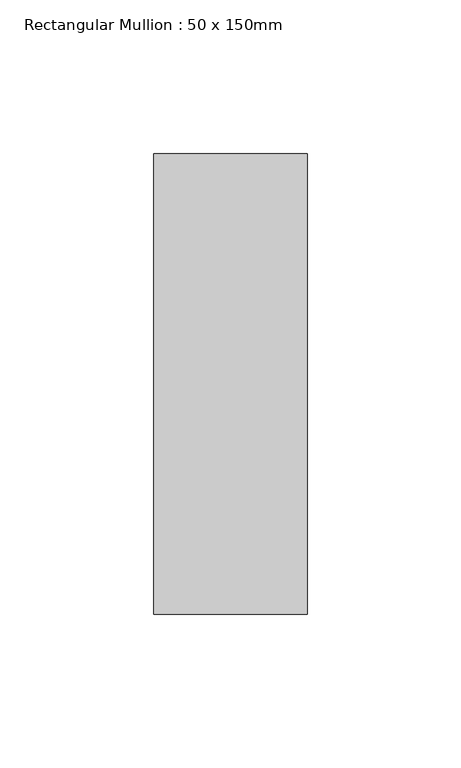
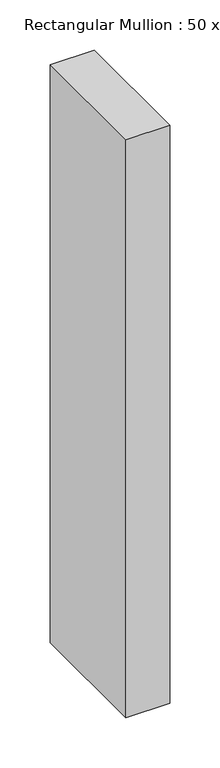
"""IFC4 building model written with IfcOpenShell, lengths in millimetres: member geometry, Rectangular Mullion : 50 x 150mm."""

import ifcopenshell
import ifcopenshell.guid

model = None  # the IFC model being written
_history = None  # IfcOwnerHistory: only IFC2X3 demands one
_inside = {}  # id of a spatial element -> (the spatial element, [elements in it])
_under = {}  # id of a project, library or spatial element -> (it, [spatial elements below it])
_declared = {}  # id of a project -> (the project, [libraries it declares])
_typed = {}  # id of a type object -> (the type object, [elements of that type])
_made_of = {}  # id of a material, layer set ... -> (it, [elements and type objects made of it])


def new_model(schema):
    """Start an empty IFC model of exactly this schema.

    Asked for "IFC4X3", IfcOpenShell would pick the latest addendum, in which some entities
    have other attributes; the version numbers below select the first issue.
    IFC2X3 requires an IfcOwnerHistory on every rooted entity: one is made here for all.
    """
    global model, _history
    if schema == "IFC4X3":
        model = ifcopenshell.file(schema_version=(4, 3, 0, 0))
    else:
        model = ifcopenshell.file(schema=schema)
    _inside.clear()
    _under.clear()
    _declared.clear()
    _typed.clear()
    _made_of.clear()
    _history = None
    if model.schema == "IFC2X3":
        org = make("IfcOrganization", Name="unknown")
        user = make(
            "IfcPersonAndOrganization",
            ThePerson=make("IfcPerson", FamilyName="unknown"),
            TheOrganization=org,
        )
        app = make(
            "IfcApplication",
            ApplicationDeveloper=org,
            Version="unknown",
            ApplicationFullName="unknown",
            ApplicationIdentifier="unknown",
        )
        _history = make(
            "IfcOwnerHistory",
            OwningUser=user,
            OwningApplication=app,
            ChangeAction="ADDED",
            CreationDate=0,
        )
    return model


def make(cls, **values):
    """One entity of the class cls with the attributes given. An attribute that is None is left unset."""
    return model.create_entity(
        cls, **{name: value for name, value in values.items() if value is not None}
    )


def rooted(cls, **values):
    """An entity with a GlobalId (a new one), such as an element, a storey or a relation."""
    return make(cls, GlobalId=ifcopenshell.guid.new(), OwnerHistory=_history, **values)


def si_unit(unit_type, name, prefix=None):
    """IfcSIUnit, for example si_unit("LENGTHUNIT", "METRE", prefix="MILLI")."""
    return make("IfcSIUnit", UnitType=unit_type, Prefix=prefix, Name=name)


def assignment(units):
    """IfcUnitAssignment: the units of a project."""
    return None if units is None else make("IfcUnitAssignment", Units=units)


def point(xyz):
    """IfcCartesianPoint."""
    return None if xyz is None else make("IfcCartesianPoint", Coordinates=xyz)


def direction(xyz):
    """IfcDirection."""
    return None if xyz is None else make("IfcDirection", DirectionRatios=xyz)


def frame(location, z_axis=None, x_axis=None):
    """IfcAxis2Placement3D, a coordinate frame: its origin and axes. An axis left out is left unset."""
    return make(
        "IfcAxis2Placement3D",
        Location=point(location),
        Axis=direction(z_axis),
        RefDirection=direction(x_axis),
    )


def origin():
    """The frame at (0, 0, 0) with its axes left unset."""
    return frame((0.0, 0.0, 0.0))


def place(relative_to, where):
    """IfcLocalPlacement: puts the frame where relative to a parent placement (None: the world)."""
    return make(
        "IfcLocalPlacement", PlacementRelTo=relative_to, RelativePlacement=where
    )


def context(
    kind, dimensions, precision=None, world=None, true_north=None, identifier=None
):
    """IfcGeometricRepresentationContext, for example the 3D "Model" context."""
    return make(
        "IfcGeometricRepresentationContext",
        ContextIdentifier=identifier,
        ContextType=kind,
        CoordinateSpaceDimension=dimensions,
        Precision=precision,
        WorldCoordinateSystem=world,
        TrueNorth=true_north,
    )


def project(units=None, contexts=None):
    """IfcProject with its units and contexts."""
    return rooted(
        "IfcProject",
        Name="project",
        RepresentationContexts=contexts,
        UnitsInContext=assignment(units),
    )


def spatial(cls, under=None, at=None, **own):
    """A site, building, storey or space (cls), placed at a placement, below another one or the project."""
    s = rooted(cls, ObjectPlacement=at, **own)
    if under is not None:
        _under.setdefault(under.id(), (under, []))[1].append(s)
    return s


def polyline(points):
    """IfcPolyline through the points."""
    return make("IfcPolyline", Points=[point(p) for p in points])


def outline(outer, holes=None, kind="AREA"):
    """IfcArbitraryClosedProfileDef: a profile drawn as a closed curve; with holes, ...WithVoids."""
    if holes is None:
        return make("IfcArbitraryClosedProfileDef", ProfileType=kind, OuterCurve=outer)
    return make(
        "IfcArbitraryProfileDefWithVoids",
        ProfileType=kind,
        OuterCurve=outer,
        InnerCurves=holes,
    )


def extrude(swept, where, along, depth):
    """IfcExtrudedAreaSolid: the profile swept, set in the frame where, extruded along a direction by depth."""
    return make(
        "IfcExtrudedAreaSolid",
        SweptArea=swept,
        Position=where,
        ExtrudedDirection=direction(along),
        Depth=depth,
    )


def shape(context_of_items, identifier, shape_type, items):
    """IfcShapeRepresentation: the items that make up one representation, for example the "Body"."""
    return make(
        "IfcShapeRepresentation",
        ContextOfItems=context_of_items,
        RepresentationIdentifier=identifier,
        RepresentationType=shape_type,
        Items=items,
    )


def source(mapping_origin, context_of_items, identifier, shape_type, items):
    """IfcRepresentationMap: a shape defined once, which mapped items show again and again."""
    return make(
        "IfcRepresentationMap",
        MappingOrigin=mapping_origin,
        MappedRepresentation=shape(context_of_items, identifier, shape_type, items),
    )


def transform(
    local_origin,
    x_axis=None,
    y_axis=None,
    z_axis=None,
    scale=None,
    scale2=None,
    scale3=None,
    uniform=True,
):
    """IfcCartesianTransformationOperator3D, or its non-uniform kind. x_axis, y_axis, z_axis: its Axis1, 2, 3."""
    if uniform:
        return make(
            "IfcCartesianTransformationOperator3D",
            Axis1=direction(x_axis),
            Axis2=direction(y_axis),
            LocalOrigin=point(local_origin),
            Scale=scale,
            Axis3=direction(z_axis),
        )
    return make(
        "IfcCartesianTransformationOperator3DnonUniform",
        Axis1=direction(x_axis),
        Axis2=direction(y_axis),
        LocalOrigin=point(local_origin),
        Scale=scale,
        Axis3=direction(z_axis),
        Scale2=scale2,
        Scale3=scale3,
    )


def mapped(mapping_source, mapping_target):
    """IfcMappedItem: shows the shape of a source again, moved by a transform."""
    return make(
        "IfcMappedItem", MappingSource=mapping_source, MappingTarget=mapping_target
    )


def made_of(thing, what):
    """Note that an element or type object is made of a material, layer set ...; save() writes the relation."""
    if what is not None:
        _made_of.setdefault(what.id(), (what, []))[1].append(thing)
    return thing


def element(
    cls,
    number,
    at=None,
    inside=None,
    cuts=None,
    type_object=None,
    material=None,
    context=None,
    identifier="Body",
    shape_type=None,
    held_by="IfcProductDefinitionShape",
    body=None,
    shapes=None,
    **own,
):
    """One element of the class cls, such as IfcWall. Its Tag is "e" and its number.

    at: its placement. inside: the storey or other place that contains it. cuts: it is an
    opening in that element (IfcRelVoidsElement). A single representation is given by context,
    identifier, shape_type and body (its items); several are given by shapes. held_by: the class
    of the entity that holds the representations. save() writes the other relations.
    """
    e = rooted(cls, Tag="e%d" % number, ObjectPlacement=at, **own)
    if body is not None:
        shapes = [shape(context, identifier, shape_type, body)]
    if shapes is not None:
        e.Representation = make(held_by, Representations=shapes)
    if inside is not None:
        _inside.setdefault(inside.id(), (inside, []))[1].append(e)
    if cuts is not None:
        rooted(
            "IfcRelVoidsElement", RelatingBuildingElement=cuts, RelatedOpeningElement=e
        )
    if type_object is not None:
        _typed.setdefault(type_object.id(), (type_object, []))[1].append(e)
    return made_of(e, material)


def aggregate(whole, parts):
    """IfcRelAggregates: a whole, such as a stair, and the parts it consists of."""
    return rooted("IfcRelAggregates", RelatingObject=whole, RelatedObjects=parts)


def save(model, path):
    """Write the relations noted so far, then the file.

    IfcRelAggregates (storeys below a building ...), IfcRelContainedInSpatialStructure (elements
    in a storey), IfcRelDefinesByType, IfcRelAssociatesMaterial and IfcRelDeclares: one each for
    every whole, place, type object, material and project.
    """
    for whole, parts in _under.values():
        aggregate(whole, parts)
    for where, things in _inside.values():
        rooted(
            "IfcRelContainedInSpatialStructure",
            RelatedElements=things,
            RelatingStructure=where,
        )
    for kind, things in _typed.values():
        rooted("IfcRelDefinesByType", RelatedObjects=things, RelatingType=kind)
    for what, things in _made_of.values():
        rooted("IfcRelAssociatesMaterial", RelatedObjects=things, RelatingMaterial=what)
    for by, libraries in _declared.values():
        rooted("IfcRelDeclares", RelatingContext=by, RelatedDefinitions=libraries)
    model.write(path)


def rectangular_mullion_50_x_150mm_205d2b36(model_context):
    return source(origin(), model_context, "Body", "SweptSolid", [
        extrude(outline(polyline([(0.0, 75.0), (0.0, -75.0), (-50.0, -75.0), (-50.0, 75.0), (0.0, 75.0)])), frame((0.0, 0.0, -700.0), z_axis=(0.0, 0.0, 1.0), x_axis=(1.0, 0.0, 0.0)), (0.0, 0.0, 1.0), 700.0),
    ])


if __name__ == "__main__":
    model = new_model("IFC4")
    model_context = context("Model", 3, world=origin())
    ifc_project = project(units=[si_unit("LENGTHUNIT", "METRE", prefix="MILLI")], contexts=[model_context])
    site = spatial("IfcSite", under=ifc_project)
    building = spatial("IfcBuilding", under=site)
    placement = place(None, origin())
    rectangular_mullion_50_x_150mm_shape = rectangular_mullion_50_x_150mm_205d2b36(model_context)
    element("IfcMember", 1, ObjectType="Rectangular Mullion : 50 x 150mm", at=placement, inside=building, context=model_context, shape_type="MappedRepresentation", body=[
        mapped(rectangular_mullion_50_x_150mm_shape, transform((0.0, 0.0, 0.0), x_axis=(1.0, 0.0, 0.0), y_axis=(0.0, 1.0, 0.0), z_axis=(0.0, 0.0, 1.0))),
    ])
    save(model, "model.ifc")

# Revit data of these elements
# Type "Rectangular Mullion : 50 x 150mm"
#   built-in parameter 1007304 = 0.492126 (stored number, unit not read)
#   built-in parameter 1007301 = 0.082021 (stored number, unit not read)
#   built-in parameter 1007300 = 0.082021 (stored number, unit not read)
# Element 1 (IfcMember, "Rectangular Mullion : 50 x 150mm")
#   Materials on its faces: "Metal - Aluminium"
# Materials
#   "Metal - Aluminium": class "Metal", colour RGB 247 247 247, transparency 0
